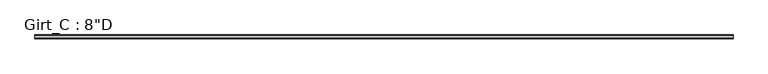
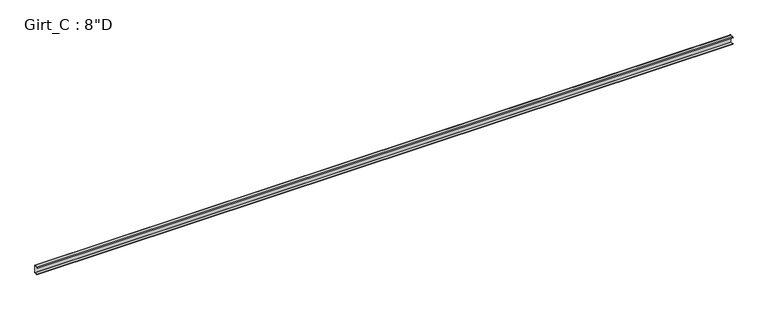
"""IFC4 building model written with IfcOpenShell, lengths in millimetres: beam geometry."""

from ifc_helpers import new_model, si_unit, point, frame, frame_2d, origin, place, context, project, spatial, polyline, circle_curve, trimmed, segment, composite_curve, outline, extrude, source, transform, mapped, element, save


def beam_e408de3d(model_context):
    return source(origin(), model_context, "Body", "SweptSolid", [
        extrude(outline(composite_curve([segment(polyline([(-87.5109375, 101.6), (-3.3734375, 101.6)]), True, "CONTINUOUS"), segment(trimmed(circle_curve(frame_2d((-3.3734375, 96.8375)), 4.7625), [point((-3.3734375, 101.6))], [point((1.3890625, 96.8375))], False, "CARTESIAN"), True, "CONTINUOUS"), segment(polyline([(1.3890625, 96.8375), (1.3890625, -96.8375)]), True, "CONTINUOUS"), segment(trimmed(circle_curve(frame_2d((-3.3734375, -96.8375)), 4.7625), [point((1.3890625, -96.8375))], [point((-3.3734375, -101.6))], False, "CARTESIAN"), True, "CONTINUOUS"), segment(polyline([(-3.3734375, -101.6), (-87.5109375, -101.6), (-99.7792647, -86.979177), (-97.6510975, -85.1934327), (-86.2154765, -98.821875), (-3.2694106, -98.821875)]), True, "CONTINUOUS"), segment(trimmed(circle_curve(frame_2d((-3.3748024, -96.8389339)), 1.9857399), [point((-3.2694106, -98.821875))], [point((-1.3890625, -96.8389339))], True, "CARTESIAN"), True, "CONTINUOUS"), segment(polyline([(-1.3890625, -96.8389339), (-1.3890625, 96.8381931)]), True, "CONTINUOUS"), segment(trimmed(circle_curve(frame_2d((-3.3741066, 96.8381931)), 1.9850441), [point((-1.3890625, 96.8381931))], [point((-3.3005807, 98.821875))], True, "CARTESIAN"), True, "CONTINUOUS"), segment(polyline([(-3.3005807, 98.821875), (-86.2154765, 98.821875), (-97.6278742, 85.221109), (-99.7560415, 87.0068534), (-87.5109375, 101.6)]), True, "CONTINUOUS")], self_intersect=False)), frame((-9154.287, 0.0, 0.0), z_axis=(1.0, 0.0, 0.0), x_axis=(0.0, 1.0, 0.0)), (0.0, 0.0, 1.0), 18371.312),
    ])


if __name__ == "__main__":
    model = new_model("IFC4")
    model_context = context("Model", 3, world=origin())
    ifc_project = project(units=[si_unit("LENGTHUNIT", "METRE", prefix="MILLI")], contexts=[model_context])
    site = spatial("IfcSite", under=ifc_project)
    building = spatial("IfcBuilding", under=site)
    placement = place(None, origin())
    beam_shape = beam_e408de3d(model_context)
    element("IfcBeam", 1, ObjectType="Girt_C : 8\"D", at=placement, inside=building, context=model_context, shape_type="MappedRepresentation", body=[
        mapped(beam_shape, transform((0.0, 0.0, 0.0), x_axis=(1.0, 0.0, 0.0), y_axis=(0.0, 1.0, 0.0), z_axis=(0.0, 0.0, 1.0))),
    ])
    save(model, "model.ifc")

# Revit data of these elements
# Type "Girt_C : 8\"D"
#   half leg = 0' - 1 3/4"
#   Web_Thickness = 0' - 0 7/64"
#   Length [instance default] = 10' - 0"
#   Leg_1 = 0' - 3 1/2"
#   Height = 0' - 8"
#   Structural Material [instance default] = none
# Element 1 (IfcBeam, "Girt_C : 8\"D")
#   Structural Material = GALVANIZED 'CEE' SECTION (8.0x3.5C - SEE STRUCT. DWGS)
#   Materials on its faces: "GALVANIZED 'CEE' SECTION (8.0x3.5C - SEE STRUCT. DWGS)"
# Materials
#   "GALVANIZED 'CEE' SECTION (8.0x3.5C - SEE STRUCT. DWGS)": class "Metal", colour RGB 137 146 153, transparency 0, Description = "Steel, mill finish", Cost = 0
